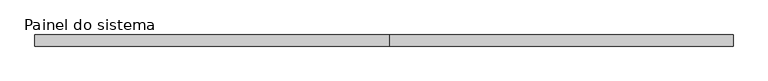
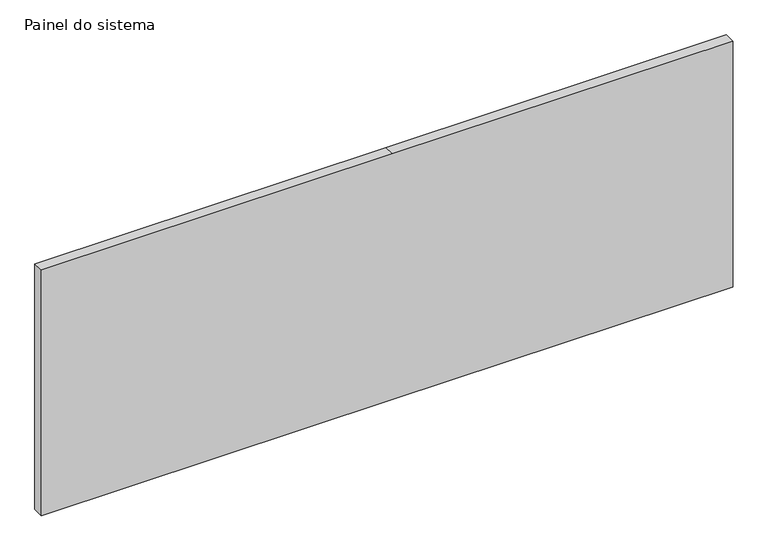
"""IFC4 building model written with IfcOpenShell, lengths in millimetres: plate geometry, Painel do sistema : Envidraçado."""

from ifc_helpers import new_model, si_unit, frame, origin, place, context, project, spatial, polyline, outline, extrude, source, transform, mapped, element, save


def painel_do_sistema_b2adb55f(model_context):
    return source(origin(), model_context, "Body", "SweptSolid", [
        extrude(outline(polyline([(0.0, -785.3166667), (0.0, 12.4999998), (0.0, 785.3166667), (590.0, 785.3166667), (590.0, 12.4999998), (590.0, -785.3166667), (0.0, -785.3166667)])), frame((0.0, -49.5, 0.0), z_axis=(0.0, 1.0, 0.0), x_axis=(0.0, 0.0, 1.0)), (0.0, 0.0, 1.0), 25.0),
    ])


if __name__ == "__main__":
    model = new_model("IFC4")
    model_context = context("Model", 3, world=origin())
    ifc_project = project(units=[si_unit("LENGTHUNIT", "METRE", prefix="MILLI")], contexts=[model_context])
    site = spatial("IfcSite", under=ifc_project)
    building = spatial("IfcBuilding", under=site)
    placement = place(None, origin())
    painel_do_sistema_shape = painel_do_sistema_b2adb55f(model_context)
    element("IfcPlate", 1, ObjectType="Painel do sistema : Envidraçado", at=placement, inside=building, context=model_context, shape_type="MappedRepresentation", body=[
        mapped(painel_do_sistema_shape, transform((0.0, 0.0, 0.0), x_axis=(1.0, 0.0, 0.0), y_axis=(0.0, 1.0, 0.0), z_axis=(0.0, 0.0, 1.0))),
    ])
    save(model, "model.ifc")

# Revit data of these elements
# Type "Painel do sistema : Envidraçado"
#   Construction Type Id = "GSP4R"
#   Analytic Construction = "Vidraça única Pilkington 1/8 pol"
#   Visual Light Transmittance = 0.9
#   Solar Heat Gain Coefficient = 0.86
#   Heat Transfer Coefficient (U) = 6.7069 W/(m²·K)
# Element 1 (IfcPlate, "Painel do sistema : Envidraçado")
#   Materials on its faces: ".VIDRO GENÉRICO"
# Materials
#   ".VIDRO GENÉRICO": class ".CC_VIDRO", colour RGB 0 128 192, transparency 0.9, Description = "Vidro comum", Cost = 0
